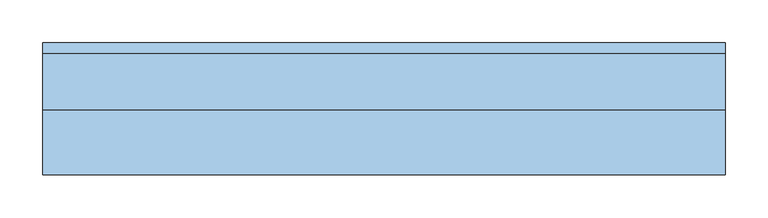
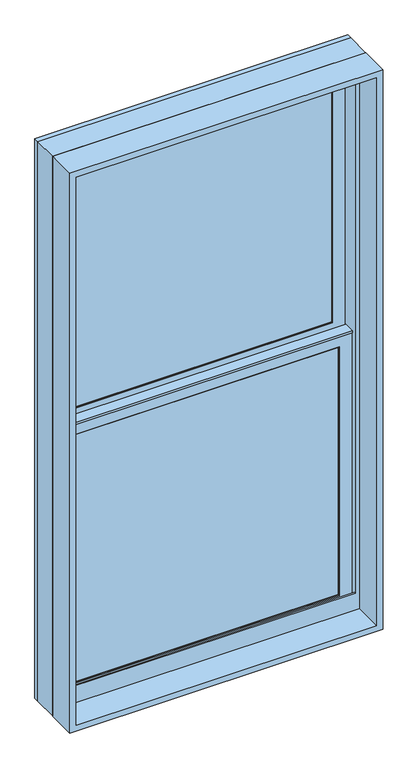
"""IFC4 building model written with IfcOpenShell, lengths in millimetres: window geometry, Window-Double_Hung-Marvin-Essential : ESDH2850."""

from ifc_helpers import new_model, si_unit, frame, origin, place, context, project, spatial, polyline, outline, extrude, faceted_brep, source, transform, mapped, element, save


def window_09f3dc34(model_context):
    return source(origin(), model_context, "Body", "SolidModel", [
        extrude(outline(polyline([(123.825, 20.6375), (123.825, 15.875), (104.775, 15.875), (104.775, 20.6375), (123.825, 20.6375)])), frame((0.0, 0.0, 984.25), z_axis=(0.0, 0.0, 1.0), x_axis=(1.0, 0.0, 0.0)), (0.0, 0.0, 1.0), 679.45),
        extrude(outline(polyline([(-104.775, 20.6375), (-104.775, 15.875), (-123.825, 15.875), (-123.825, 20.6375), (-104.775, 20.6375)])), frame((0.0, 0.0, 984.25), z_axis=(0.0, 0.0, 1.0), x_axis=(1.0, 0.0, 0.0)), (0.0, 0.0, 1.0), 679.45),
        extrude(outline(polyline([(342.9, 20.6375), (342.9, 15.875), (-342.9, 15.875), (-342.9, 20.6375), (342.9, 20.6375)])), frame((0.0, 0.0, 1314.45), z_axis=(0.0, 0.0, 1.0), x_axis=(1.0, 0.0, 0.0)), (0.0, 0.0, 1.0), 19.05),
        extrude(outline(polyline([(-123.825, 46.83125), (-123.825, 51.59375), (-104.775, 51.59375), (-104.775, 46.83125), (-123.825, 46.83125)])), frame((0.0, 0.0, 1701.8), z_axis=(0.0, 0.0, 1.0), x_axis=(1.0, 0.0, 0.0)), (0.0, 0.0, 1.0), 679.45),
        extrude(outline(polyline([(104.775, 46.83125), (104.775, 51.59375), (123.825, 51.59375), (123.825, 46.83125), (104.775, 46.83125)])), frame((0.0, 0.0, 1701.8), z_axis=(0.0, 0.0, 1.0), x_axis=(1.0, 0.0, 0.0)), (0.0, 0.0, 1.0), 679.45),
        extrude(outline(polyline([(-342.9, 46.83125), (-342.9, 51.59375), (342.9, 51.59375), (342.9, 46.83125), (-342.9, 46.83125)])), frame((0.0, 0.0, 2032.0), z_axis=(0.0, 0.0, 1.0), x_axis=(1.0, 0.0, 0.0)), (0.0, 0.0, 1.0), 19.05),
        extrude(outline(polyline([(123.825, 20.6375), (104.775, 20.6375), (104.775, 25.4), (123.825, 25.4), (123.825, 20.6375)])), frame((0.0, 0.0, 984.25), z_axis=(0.0, 0.0, 1.0), x_axis=(1.0, 0.0, 0.0)), (0.0, 0.0, 1.0), 679.45),
        extrude(outline(polyline([(-104.775, 20.6375), (-123.825, 20.6375), (-123.825, 25.4), (-104.775, 25.4), (-104.775, 20.6375)])), frame((0.0, 0.0, 984.25), z_axis=(0.0, 0.0, 1.0), x_axis=(1.0, 0.0, 0.0)), (0.0, 0.0, 1.0), 679.45),
        extrude(outline(polyline([(342.9, 20.6375), (-342.9, 20.6375), (-342.9, 25.4), (342.9, 25.4), (342.9, 20.6375)])), frame((0.0, 0.0, 1314.45), z_axis=(0.0, 0.0, 1.0), x_axis=(1.0, 0.0, 0.0)), (0.0, 0.0, 1.0), 19.05),
        extrude(outline(polyline([(-123.825, 56.35625), (-104.775, 56.35625), (-104.775, 51.59375), (-123.825, 51.59375), (-123.825, 56.35625)])), frame((0.0, 0.0, 1701.8), z_axis=(0.0, 0.0, 1.0), x_axis=(1.0, 0.0, 0.0)), (0.0, 0.0, 1.0), 679.45),
        extrude(outline(polyline([(104.775, 56.35625), (123.825, 56.35625), (123.825, 51.59375), (104.775, 51.59375), (104.775, 56.35625)])), frame((0.0, 0.0, 1701.8), z_axis=(0.0, 0.0, 1.0), x_axis=(1.0, 0.0, 0.0)), (0.0, 0.0, 1.0), 679.45),
        extrude(outline(polyline([(-342.9, 56.35625), (342.9, 56.35625), (342.9, 51.59375), (-342.9, 51.59375), (-342.9, 56.35625)])), frame((0.0, 0.0, 2032.0), z_axis=(0.0, 0.0, 1.0), x_axis=(1.0, 0.0, 0.0)), (0.0, 0.0, 1.0), 19.05),
        faceted_brep([(-369.8875, 5.6780605, 1693.7351748), (-369.8875, 5.6780605, 1689.1), (369.8875, 5.6780605, 1689.1), (369.8875, 5.6780605, 1693.7351748), (-369.8875, 34.8118605, 1693.7351748), (369.8875, 34.8118605, 1693.7351748), (369.8875, 34.8118605, 1689.1), (-369.8875, 34.8118605, 1689.1), (-369.8875, 30.1625, 1689.1), (-369.8875, 30.1625, 957.2625), (-369.8875, 8.9241104, 957.2625), (-369.8875, 8.9241104, 1689.1), (369.8875, 8.9241104, 1689.1), (369.8875, 30.1625, 1689.1), (369.8875, 8.9241104, 957.2625), (369.8875, 30.1625, 957.2625), (-354.0034752, 11.90625, 1674.8034752), (-354.0034752, 30.1625, 1674.8034752), (354.0034752, 30.1625, 1674.8034752), (354.0034752, 11.90625, 1674.8034752), (-337.34375, 10.4662439, 1658.14375), (-337.34375, 11.90625, 1658.14375), (337.34375, 11.90625, 1658.14375), (337.34375, 10.4662439, 1658.14375), (338.8858834, 8.9241104, 1659.6858834), (-338.8858834, 8.9241104, 1659.6858834), (354.0034752, 30.1625, 973.1465248), (354.0034752, 11.90625, 973.1465248), (337.34375, 11.90625, 989.80625), (337.34375, 10.4662439, 989.80625), (338.8858834, 8.9241104, 988.2641166), (-354.0034752, 30.1625, 973.1465248), (-354.0034752, 11.90625, 973.1465248), (-337.34375, 11.90625, 989.80625), (-337.34375, 10.4662439, 989.80625), (-338.8858834, 8.9241104, 988.2641166)], [[[0, 1, 2, 3]], [[4, 5, 6, 7]], [[1, 0, 4, 7, 8, 9, 10, 11]], [[2, 1, 11, 12]], [[7, 6, 13, 8]], [[3, 2, 12, 14, 15, 13, 6, 5]], [[0, 3, 5, 4]], [[16, 17, 18, 19]], [[20, 21, 22, 23]], [[20, 23, 24, 25]], [[19, 18, 26, 27]], [[23, 22, 28, 29]], [[24, 23, 29, 30]], [[27, 26, 31, 32]], [[29, 28, 33, 34]], [[30, 29, 34, 35]], [[15, 14, 10, 9]], [[15, 9, 8, 13], [18, 17, 31, 26]], [[17, 16, 32, 31]], [[16, 19, 27, 32], [22, 21, 33, 28]], [[21, 20, 34, 33]], [[20, 25, 35, 34]], [[10, 14, 12, 11], [25, 24, 30, 35]]]),
        extrude(outline(polyline([(38.5955581, 1674.8125), (33.5778968, 1674.8125), (33.5778968, 1676.4), (39.9405976, 1676.4), (39.9405976, 1674.8125), (61.515625, 1674.8125), (47.6307501, 1671.4975159), (38.5955581, 1671.4975159), (38.5955581, 1674.8125)])), frame((-369.8875, 0.0, 0.0), z_axis=(1.0, 0.0, 0.0), x_axis=(0.0, 1.0, 0.0)), (0.0, 0.0, 1.0), 739.775),
        faceted_brep([(400.05, 0.0, 927.1), (400.05, 0.0, 2438.4), (-400.05, 0.0, 2438.4), (-400.05, 0.0, 927.1), (373.85625, 0.0, 988.21875), (-373.85625, 0.0, 988.21875), (-373.85625, 0.0, 2412.20625), (373.85625, 0.0, 2412.20625), (373.85625, 3.96875, 927.1), (-373.85625, 3.96875, 927.1), (-373.85625, 3.96875, 988.21875), (373.85625, 3.96875, 988.21875), (-400.05, 65.6828125, 927.1), (-373.85625, 65.6828125, 927.1), (373.85625, 65.6828125, 927.1), (400.05, 65.6828125, 927.1), (-400.05, 65.6828125, 2438.4), (400.05, 65.6828125, 2438.4), (373.85625, 65.6828125, 2412.20625), (-373.85625, 65.6828125, 2412.20625)], [[[0, 1, 2, 3], [4, 5, 6, 7]], [[8, 9, 10, 11]], [[5, 4, 11, 10]], [[0, 3, 12, 13, 9, 8, 14, 15]], [[13, 12, 16, 17, 15, 14, 18, 19]], [[13, 19, 6, 5, 10, 9]], [[7, 6, 19, 18]], [[18, 14, 8, 11, 4, 7]], [[1, 0, 15, 17]], [[2, 1, 17, 16]], [[3, 2, 16, 12]]]),
        faceted_brep([(373.85625, 30.1625, 1682.75), (372.26875, 30.1625, 1682.75), (372.26875, 30.1625, 951.4544613), (373.85625, 30.1625, 951.4544613), (-372.26875, 30.1625, 1682.75), (-373.85625, 30.1625, 1682.75), (-373.85625, 30.1625, 951.4544613), (-372.26875, 30.1625, 951.4544613), (372.26875, 63.5, 1682.75), (373.85625, 63.5, 1682.75), (373.85625, 63.5, 944.9743077), (372.26875, 63.5, 944.9743077), (-373.85625, 63.5, 1682.75), (-372.26875, 63.5, 1682.75), (-372.26875, 63.5, 944.9743077), (-373.85625, 63.5, 944.9743077), (385.1108932, 3.96875, 956.5460105), (385.1108932, 3.96875, 927.1), (385.1108932, 65.6828125, 927.1), (385.1108932, 65.6828125, 944.550012), (-385.1108932, 3.96875, 927.1), (-385.1108932, 3.96875, 956.5460105), (-385.1108932, 65.6828125, 944.550012), (-385.1108932, 65.6828125, 927.1), (385.1108932, 78.58125, 942.0428097), (-385.1108932, 78.58125, 942.0428097), (-383.0971252, 68.2348864, 944.0539391), (-365.13135, 68.2348864, 944.0539391), (-365.13135, 65.6828125, 944.550012), (365.13135, 65.6828125, 944.550012), (365.13135, 68.2348864, 944.0539391), (383.0971252, 68.2348864, 944.0539391), (-400.05, 65.6828125, 927.1), (-400.05, 78.5948249, 927.1), (400.05, 78.5948249, 927.1), (400.05, 65.6828125, 927.1), (-400.05, 78.58125, 2438.4), (400.05, 78.58125, 2438.4), (385.1108932, 78.58125, 2423.4608932), (-385.1108932, 78.58125, 2423.4608932), (-400.05, 65.6828125, 2438.4), (-383.0971252, 68.2348864, 2421.4471252), (383.0971252, 68.2348864, 2421.4471252), (365.13135, 68.2348864, 2403.48135), (-365.13135, 68.2348864, 2403.48135), (-365.13135, 65.6828125, 2403.48135), (365.13135, 65.6828125, 2403.48135), (400.05, 65.6828125, 2438.4)], [[[0, 1, 2, 3]], [[4, 5, 6, 7]], [[8, 9, 10, 11]], [[12, 13, 14, 15]], [[1, 8, 11, 2]], [[9, 0, 3, 10]], [[1, 0, 9, 8]], [[5, 4, 13, 12]], [[5, 12, 15, 6]], [[13, 4, 7, 14]], [[16, 17, 18, 19]], [[20, 21, 22, 23]], [[24, 25, 26, 27, 28, 22, 21, 16, 19, 29, 30, 31], [3, 2, 11, 10], [7, 6, 15, 14]], [[17, 16, 21, 20]], [[17, 20, 23, 32, 33, 34, 35, 18]], [[34, 33, 36, 37], [25, 24, 38, 39]], [[33, 32, 40, 36]], [[39, 41, 26, 25]], [[41, 42, 31, 30, 43, 44, 27, 26]], [[44, 45, 28, 27]], [[40, 32, 23, 22, 28, 45, 46, 29, 19, 18, 35, 47]], [[36, 40, 47, 37]], [[39, 38, 42, 41]], [[44, 43, 46, 45]], [[34, 37, 47, 35]], [[42, 38, 24, 31]], [[46, 43, 30, 29]]]),
        extrude(outline(polyline([(350.04375, 11.90625), (-350.04375, 11.90625), (-350.04375, 15.08125), (350.04375, 15.08125), (350.04375, 11.90625)])), frame((0.0, 0.0, 977.10625), z_axis=(0.0, 0.0, 1.0), x_axis=(1.0, 0.0, 0.0)), (0.0, 0.0, 1.0), 693.7375),
        extrude(outline(polyline([(350.04375, 42.8625), (-350.04375, 42.8625), (-350.04375, 46.0375), (350.04375, 46.0375), (350.04375, 42.8625)])), frame((0.0, 0.0, 1694.65625), z_axis=(0.0, 0.0, 1.0), x_axis=(1.0, 0.0, 0.0)), (0.0, 0.0, 1.0), 693.7375),
        faceted_brep([(-337.34375, 31.194477, 1658.14375), (-338.8858834, 32.7366104, 1659.6858834), (338.8858834, 32.7366104, 1659.6858834), (337.34375, 31.194477, 1658.14375), (-337.34375, 30.1625, 1658.14375), (337.34375, 30.1625, 1658.14375), (-369.8875, 32.7366104, 1690.6875), (-369.8875, 30.1625, 1690.6875), (369.8875, 30.1625, 1690.6875), (369.8875, 32.7366104, 1690.6875), (338.8858834, 32.7366104, 988.2641166), (337.34375, 31.194477, 989.80625), (337.34375, 30.1625, 989.80625), (369.8875, 30.1625, 957.2625), (369.8875, 32.7366104, 957.2625), (-338.8858834, 32.7366104, 988.2641166), (-337.34375, 31.194477, 989.80625), (-337.34375, 30.1625, 989.80625), (-369.8875, 30.1625, 957.2625), (-369.8875, 32.7366104, 957.2625)], [[[0, 1, 2, 3]], [[4, 0, 3, 5]], [[6, 7, 8, 9]], [[3, 2, 10, 11]], [[5, 3, 11, 12]], [[9, 8, 13, 14]], [[11, 10, 15, 16]], [[12, 11, 16, 17]], [[14, 13, 18, 19]], [[9, 14, 19, 6], [1, 15, 10, 2]], [[16, 15, 1, 0]], [[17, 16, 0, 4]], [[7, 18, 13, 8], [5, 12, 17, 4]], [[19, 18, 7, 6]]]),
        faceted_brep([(-354.0034752, 42.8625, 2392.3534752), (-354.0034752, 61.11875, 2392.3534752), (354.0034752, 61.11875, 2392.3534752), (354.0034752, 42.8625, 2392.3534752), (-337.34375, 41.4224939, 2375.69375), (-337.34375, 42.8625, 2375.69375), (337.34375, 42.8625, 2375.69375), (337.34375, 41.4224939, 2375.69375), (-338.8858834, 39.8803604, 2377.2358834), (338.8858834, 39.8803604, 2377.2358834), (-369.8875, 61.11875, 2408.2375), (-369.8875, 39.8803604, 2408.2375), (369.8875, 39.8803604, 2408.2375), (369.8875, 61.11875, 2408.2375), (354.0034752, 61.11875, 1690.6965248), (354.0034752, 42.8625, 1690.6965248), (337.34375, 42.8625, 1707.35625), (337.34375, 41.4224939, 1707.35625), (338.8858834, 39.8803604, 1705.8141166), (369.8875, 39.8803604, 1674.8125), (369.8875, 61.11875, 1674.8125), (-354.0034752, 61.11875, 1690.6965248), (-354.0034752, 42.8625, 1690.6965248), (-337.34375, 42.8625, 1707.35625), (-337.34375, 41.4224939, 1707.35625), (-338.8858834, 39.8803604, 1705.8141166), (-369.8875, 39.8803604, 1674.8125), (-369.8875, 61.11875, 1674.8125)], [[[0, 1, 2, 3]], [[4, 5, 6, 7]], [[8, 4, 7, 9]], [[10, 11, 12, 13]], [[3, 2, 14, 15]], [[7, 6, 16, 17]], [[9, 7, 17, 18]], [[13, 12, 19, 20]], [[15, 14, 21, 22]], [[17, 16, 23, 24]], [[18, 17, 24, 25]], [[20, 19, 26, 27]], [[13, 20, 27, 10], [1, 21, 14, 2]], [[22, 21, 1, 0]], [[3, 15, 22, 0], [5, 23, 16, 6]], [[24, 23, 5, 4]], [[25, 24, 4, 8]], [[11, 26, 19, 12], [9, 18, 25, 8]], [[27, 26, 11, 10]]]),
        faceted_brep([(-369.8875, 61.11875, 1674.8125), (-369.8875, 63.6928604, 1674.8125), (369.8875, 63.6928604, 1674.8125), (369.8875, 61.11875, 1674.8125), (-337.34375, 62.150727, 1707.35625), (-337.34375, 61.11875, 1707.35625), (337.34375, 61.11875, 1707.35625), (337.34375, 62.150727, 1707.35625), (-338.8858834, 63.6928604, 1705.8141166), (338.8858834, 63.6928604, 1705.8141166), (369.8875, 63.6928604, 2408.2375), (369.8875, 61.11875, 2408.2375), (337.34375, 61.11875, 2375.69375), (337.34375, 62.150727, 2375.69375), (338.8858834, 63.6928604, 2377.2358834), (-369.8875, 63.6928604, 2408.2375), (-369.8875, 61.11875, 2408.2375), (-337.34375, 61.11875, 2375.69375), (-337.34375, 62.150727, 2375.69375), (-338.8858834, 63.6928604, 2377.2358834)], [[[0, 1, 2, 3]], [[4, 5, 6, 7]], [[8, 4, 7, 9]], [[3, 2, 10, 11]], [[7, 6, 12, 13]], [[9, 7, 13, 14]], [[11, 10, 15, 16]], [[13, 12, 17, 18]], [[14, 13, 18, 19]], [[16, 15, 1, 0]], [[3, 11, 16, 0], [5, 17, 12, 6]], [[18, 17, 5, 4]], [[19, 18, 4, 8]], [[1, 15, 10, 2], [9, 14, 19, 8]]]),
        extrude(outline(polyline([(350.04375, 26.19375), (-350.04375, 26.19375), (-350.04375, 30.1625), (350.04375, 30.1625), (350.04375, 26.19375)])), frame((0.0, 0.0, 977.10625), z_axis=(0.0, 0.0, 1.0), x_axis=(1.0, 0.0, 0.0)), (0.0, 0.0, 1.0), 693.7375),
        extrude(outline(polyline([(350.04375, 57.15), (-350.04375, 57.15), (-350.04375, 61.11875), (350.04375, 61.11875), (350.04375, 57.15)])), frame((0.0, 0.0, 1694.65625), z_axis=(0.0, 0.0, 1.0), x_axis=(1.0, 0.0, 0.0)), (0.0, 0.0, 1.0), 693.7375),
        extrude(outline(polyline([(2438.4, 400.05), (2438.4, -400.05), (927.1, -400.05), (927.1, 400.05), (2438.4, 400.05)]), holes=[polyline([(2422.525, 384.175), (942.975, 384.175), (942.975, -384.175), (2422.525, -384.175), (2422.525, 384.175)])]), frame((0.0, -76.2, 0.0), z_axis=(0.0, 1.0, 0.0), x_axis=(0.0, 0.0, 1.0)), (0.0, 0.0, 1.0), 75.40625),
    ])


if __name__ == "__main__":
    model = new_model("IFC4")
    model_context = context("Model", 3, world=origin())
    ifc_project = project(units=[si_unit("LENGTHUNIT", "METRE", prefix="MILLI")], contexts=[model_context])
    site = spatial("IfcSite", under=ifc_project)
    building = spatial("IfcBuilding", under=site)
    placement = place(None, origin())
    window_shape = window_09f3dc34(model_context)
    element("IfcWindow", 1, ObjectType="Window-Double_Hung-Marvin-Essential : ESDH2850", at=placement, inside=building, context=model_context, shape_type="MappedRepresentation", body=[
        mapped(window_shape, transform((0.0, 0.0, 0.0), x_axis=(1.0, 0.0, 0.0), y_axis=(0.0, 1.0, 0.0), z_axis=(0.0, 0.0, 1.0))),
    ])
    save(model, "model.ifc")

# Revit data of these elements
# Type "Window-Double_Hung-Marvin-Essential : ESDH2850"
#   Type Mark = "64"
#   Window Type = "Essential Double Hung"
#   Product data url = "https://bimobject.com/marvin-windows-and-doors/product/marvin-dhwau"
#   Product Guid = "c4a96547-874c-4385-91dc-a058adc19d98"
#   Frame = "All Ultrex"
#   Egress Window = "No"
#   URL = "www.marvin.com"
#   Model = "ESDH2850"
#   Manufacturer = "Marvin Windows and Doors"
#   Label Egress = ""
#   Glass Type = "IG Low E II with Argon"
#   Design Pressure = "DP50"
#   Description = "3260 DBHG"
#   Analytic Construction = "<None>"
#   Prairie Corner Width = 0' - 4"
#   Prairie Corner Height = 0' - 4"
#   Egress Width = 2' - 4 9/16"
#   Egress Height = 2' - 1 27/128"
#   Rough Width = 2' - 8"
#   Rough Height = 5' - 0"
#   Nominal Width = 2' - 8"
#   Nominal Height = 5' - 0"
#   Inset to Installation Flange [instance default] = 0' - 1"
#   Height = 4' - 11 1/2"
#   Egress Area = 5.00061 SF
#   Default Head Height = 8' - 0"
#   Width = 2' - 7 1/2"
#   Daylight Area = 9.7073 SF
#   DLO Width = 2' - 2 9/16"
#   DLO Height = 2' - 2 5/16"
#   Muntins Top Sash = yes
#   Lites Wide Top Sash = 3
#   Lites Wide Bottom Sash = 3
#   Lites High Top Sash = 2
#   Lites High Bottom Sash = 2
#   Lite Cut Prairie 9 = no
#   Lite Cut HV Grid = yes
#   Muntins Bottom Sash = yes
#   Label Visibility = no
#   Jamb Extension Visibility = yes
#   Edition number = 1
#   Interior Material = Ultrex-Marvin-Stonewhite
#   Glazing Material = Glass-Marvin-IG Low E II with Argon
#   Cladding Material = Ultrex-Marvin-Pebblegray
#   Wall Closure = (empty or 0)
#   Assembly Code = ""
# Element 1 (IfcWindow, "Window-Double_Hung-Marvin-Essential : ESDH2850")
#   Materials on its faces: "Ultrex-Marvin-Pebblegray", "Ultrex-Marvin-Stonewhite", "Glass-Marvin-IG Low E II with Argon"
# Materials
#   "Ultrex-Marvin-Stonewhite": class "Paint", colour RGB 250 251 245, transparency 0
#   "Glass-Marvin-IG Low E II with Argon": class "Glass", colour RGB 0 128 192, transparency 0.85
#   "Ultrex-Marvin-Pebblegray": class "Paint", colour RGB 189 185 173, transparency 0
